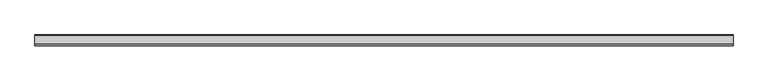
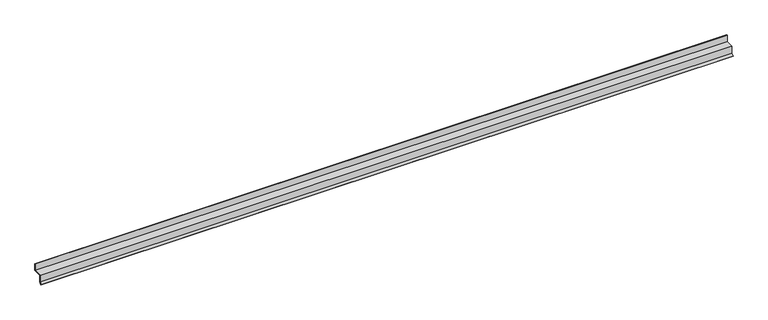
"""IFC4 building model written with IfcOpenShell, lengths in millimetres: proxy geometry, Generic Models 7:Generic Models 1:337419:Generic Models 1:337419 : Generic Models 7:Generic Models 1:337419:7 : Generic Models 7:Generic Models 1:337419:Generic Models 1:337419 : Generic Models 7:Generic Models 1:337419:301336."""

import ifcopenshell
import ifcopenshell.guid

model = None  # the IFC model being written
_history = None  # IfcOwnerHistory: only IFC2X3 demands one
_inside = {}  # id of a spatial element -> (the spatial element, [elements in it])
_under = {}  # id of a project, library or spatial element -> (it, [spatial elements below it])
_declared = {}  # id of a project -> (the project, [libraries it declares])
_typed = {}  # id of a type object -> (the type object, [elements of that type])
_made_of = {}  # id of a material, layer set ... -> (it, [elements and type objects made of it])


def new_model(schema):
    """Start an empty IFC model of exactly this schema.

    Asked for "IFC4X3", IfcOpenShell would pick the latest addendum, in which some entities
    have other attributes; the version numbers below select the first issue.
    IFC2X3 requires an IfcOwnerHistory on every rooted entity: one is made here for all.
    """
    global model, _history
    if schema == "IFC4X3":
        model = ifcopenshell.file(schema_version=(4, 3, 0, 0))
    else:
        model = ifcopenshell.file(schema=schema)
    _inside.clear()
    _under.clear()
    _declared.clear()
    _typed.clear()
    _made_of.clear()
    _history = None
    if model.schema == "IFC2X3":
        org = make("IfcOrganization", Name="unknown")
        user = make(
            "IfcPersonAndOrganization",
            ThePerson=make("IfcPerson", FamilyName="unknown"),
            TheOrganization=org,
        )
        app = make(
            "IfcApplication",
            ApplicationDeveloper=org,
            Version="unknown",
            ApplicationFullName="unknown",
            ApplicationIdentifier="unknown",
        )
        _history = make(
            "IfcOwnerHistory",
            OwningUser=user,
            OwningApplication=app,
            ChangeAction="ADDED",
            CreationDate=0,
        )
    return model


def make(cls, **values):
    """One entity of the class cls with the attributes given. An attribute that is None is left unset."""
    return model.create_entity(
        cls, **{name: value for name, value in values.items() if value is not None}
    )


def rooted(cls, **values):
    """An entity with a GlobalId (a new one), such as an element, a storey or a relation."""
    return make(cls, GlobalId=ifcopenshell.guid.new(), OwnerHistory=_history, **values)


def si_unit(unit_type, name, prefix=None):
    """IfcSIUnit, for example si_unit("LENGTHUNIT", "METRE", prefix="MILLI")."""
    return make("IfcSIUnit", UnitType=unit_type, Prefix=prefix, Name=name)


def assignment(units):
    """IfcUnitAssignment: the units of a project."""
    return None if units is None else make("IfcUnitAssignment", Units=units)


def point(xyz):
    """IfcCartesianPoint."""
    return None if xyz is None else make("IfcCartesianPoint", Coordinates=xyz)


def direction(xyz):
    """IfcDirection."""
    return None if xyz is None else make("IfcDirection", DirectionRatios=xyz)


def frame(location, z_axis=None, x_axis=None):
    """IfcAxis2Placement3D, a coordinate frame: its origin and axes. An axis left out is left unset."""
    return make(
        "IfcAxis2Placement3D",
        Location=point(location),
        Axis=direction(z_axis),
        RefDirection=direction(x_axis),
    )


def origin():
    """The frame at (0, 0, 0) with its axes left unset."""
    return frame((0.0, 0.0, 0.0))


def place(relative_to, where):
    """IfcLocalPlacement: puts the frame where relative to a parent placement (None: the world)."""
    return make(
        "IfcLocalPlacement", PlacementRelTo=relative_to, RelativePlacement=where
    )


def context(
    kind, dimensions, precision=None, world=None, true_north=None, identifier=None
):
    """IfcGeometricRepresentationContext, for example the 3D "Model" context."""
    return make(
        "IfcGeometricRepresentationContext",
        ContextIdentifier=identifier,
        ContextType=kind,
        CoordinateSpaceDimension=dimensions,
        Precision=precision,
        WorldCoordinateSystem=world,
        TrueNorth=true_north,
    )


def project(units=None, contexts=None):
    """IfcProject with its units and contexts."""
    return rooted(
        "IfcProject",
        Name="project",
        RepresentationContexts=contexts,
        UnitsInContext=assignment(units),
    )


def spatial(cls, under=None, at=None, **own):
    """A site, building, storey or space (cls), placed at a placement, below another one or the project."""
    s = rooted(cls, ObjectPlacement=at, **own)
    if under is not None:
        _under.setdefault(under.id(), (under, []))[1].append(s)
    return s


def polyline(points):
    """IfcPolyline through the points."""
    return make("IfcPolyline", Points=[point(p) for p in points])


def outline(outer, holes=None, kind="AREA"):
    """IfcArbitraryClosedProfileDef: a profile drawn as a closed curve; with holes, ...WithVoids."""
    if holes is None:
        return make("IfcArbitraryClosedProfileDef", ProfileType=kind, OuterCurve=outer)
    return make(
        "IfcArbitraryProfileDefWithVoids",
        ProfileType=kind,
        OuterCurve=outer,
        InnerCurves=holes,
    )


def extrude(swept, where, along, depth):
    """IfcExtrudedAreaSolid: the profile swept, set in the frame where, extruded along a direction by depth."""
    return make(
        "IfcExtrudedAreaSolid",
        SweptArea=swept,
        Position=where,
        ExtrudedDirection=direction(along),
        Depth=depth,
    )


def shape(context_of_items, identifier, shape_type, items):
    """IfcShapeRepresentation: the items that make up one representation, for example the "Body"."""
    return make(
        "IfcShapeRepresentation",
        ContextOfItems=context_of_items,
        RepresentationIdentifier=identifier,
        RepresentationType=shape_type,
        Items=items,
    )


def source(mapping_origin, context_of_items, identifier, shape_type, items):
    """IfcRepresentationMap: a shape defined once, which mapped items show again and again."""
    return make(
        "IfcRepresentationMap",
        MappingOrigin=mapping_origin,
        MappedRepresentation=shape(context_of_items, identifier, shape_type, items),
    )


def transform(
    local_origin,
    x_axis=None,
    y_axis=None,
    z_axis=None,
    scale=None,
    scale2=None,
    scale3=None,
    uniform=True,
):
    """IfcCartesianTransformationOperator3D, or its non-uniform kind. x_axis, y_axis, z_axis: its Axis1, 2, 3."""
    if uniform:
        return make(
            "IfcCartesianTransformationOperator3D",
            Axis1=direction(x_axis),
            Axis2=direction(y_axis),
            LocalOrigin=point(local_origin),
            Scale=scale,
            Axis3=direction(z_axis),
        )
    return make(
        "IfcCartesianTransformationOperator3DnonUniform",
        Axis1=direction(x_axis),
        Axis2=direction(y_axis),
        LocalOrigin=point(local_origin),
        Scale=scale,
        Axis3=direction(z_axis),
        Scale2=scale2,
        Scale3=scale3,
    )


def mapped(mapping_source, mapping_target):
    """IfcMappedItem: shows the shape of a source again, moved by a transform."""
    return make(
        "IfcMappedItem", MappingSource=mapping_source, MappingTarget=mapping_target
    )


def made_of(thing, what):
    """Note that an element or type object is made of a material, layer set ...; save() writes the relation."""
    if what is not None:
        _made_of.setdefault(what.id(), (what, []))[1].append(thing)
    return thing


def element(
    cls,
    number,
    at=None,
    inside=None,
    cuts=None,
    type_object=None,
    material=None,
    context=None,
    identifier="Body",
    shape_type=None,
    held_by="IfcProductDefinitionShape",
    body=None,
    shapes=None,
    **own,
):
    """One element of the class cls, such as IfcWall. Its Tag is "e" and its number.

    at: its placement. inside: the storey or other place that contains it. cuts: it is an
    opening in that element (IfcRelVoidsElement). A single representation is given by context,
    identifier, shape_type and body (its items); several are given by shapes. held_by: the class
    of the entity that holds the representations. save() writes the other relations.
    """
    e = rooted(cls, Tag="e%d" % number, ObjectPlacement=at, **own)
    if body is not None:
        shapes = [shape(context, identifier, shape_type, body)]
    if shapes is not None:
        e.Representation = make(held_by, Representations=shapes)
    if inside is not None:
        _inside.setdefault(inside.id(), (inside, []))[1].append(e)
    if cuts is not None:
        rooted(
            "IfcRelVoidsElement", RelatingBuildingElement=cuts, RelatedOpeningElement=e
        )
    if type_object is not None:
        _typed.setdefault(type_object.id(), (type_object, []))[1].append(e)
    return made_of(e, material)


def aggregate(whole, parts):
    """IfcRelAggregates: a whole, such as a stair, and the parts it consists of."""
    return rooted("IfcRelAggregates", RelatingObject=whole, RelatedObjects=parts)


def save(model, path):
    """Write the relations noted so far, then the file.

    IfcRelAggregates (storeys below a building ...), IfcRelContainedInSpatialStructure (elements
    in a storey), IfcRelDefinesByType, IfcRelAssociatesMaterial and IfcRelDeclares: one each for
    every whole, place, type object, material and project.
    """
    for whole, parts in _under.values():
        aggregate(whole, parts)
    for where, things in _inside.values():
        rooted(
            "IfcRelContainedInSpatialStructure",
            RelatedElements=things,
            RelatingStructure=where,
        )
    for kind, things in _typed.values():
        rooted("IfcRelDefinesByType", RelatedObjects=things, RelatingType=kind)
    for what, things in _made_of.values():
        rooted("IfcRelAssociatesMaterial", RelatedObjects=things, RelatingMaterial=what)
    for by, libraries in _declared.values():
        rooted("IfcRelDeclares", RelatingContext=by, RelatedDefinitions=libraries)
    model.write(path)


def generic_models_4a6affe0(model_context):
    return source(origin(), model_context, "Body", "SweptSolid", [
        extrude(outline(polyline([(-568211.286182, 4851.0990819), (-568271.214307, 4851.0990819), (-568271.214307, 4801.9264699), (-568285.4983852, 4787.6423917), (-568287.4628162, 4789.6068227), (-568273.992432, 4803.0772069), (-568273.992432, 4853.8772069), (-568214.064307, 4853.8772069), (-568214.064307, 4901.8990819), (-568211.286182, 4901.8990819), (-568211.286182, 4851.0990819)])), frame((591306.0367242, 0.0, 0.0), z_axis=(1.0, 0.0, 0.0), x_axis=(0.0, 1.0, 0.0)), (0.0, 0.0, 1.0), 4876.8),
    ])


if __name__ == "__main__":
    model = new_model("IFC4")
    model_context = context("Model", 3, world=origin())
    ifc_project = project(units=[si_unit("LENGTHUNIT", "METRE", prefix="MILLI")], contexts=[model_context])
    site = spatial("IfcSite", under=ifc_project)
    building = spatial("IfcBuilding", under=site)
    placement = place(None, origin())
    generic_models_shape = generic_models_4a6affe0(model_context)
    element("IfcBuildingElementProxy", 1, Name="Generic Models 7:Generic Models 1:337419:Generic Models 1:337419 : Generic Models 7:Generic Models 1:337419:7 : Generic Models 7:Generic Models 1:337419:Generic Models 1:337419 : Generic Models 7:Generic Models 1:337419:301336", ObjectType="Generic Models 7:Generic Models 1:337419:Generic Models 1:337419 : Generic Models 7:Generic Models 1:337419:7 : Generic Models 7:Generic Models 1:337419:Generic Models 1:337419 : Generic Models 7:Generic Models 1:337419:301336", at=placement, inside=building, context=model_context, shape_type="MappedRepresentation", body=[
        mapped(generic_models_shape, transform((0.0, 0.0, 0.0), x_axis=(1.0, 0.0, 0.0), y_axis=(0.0, 1.0, 0.0), z_axis=(0.0, 0.0, 1.0))),
    ])
    save(model, "model.ifc")

# Revit data of these elements
# Type "Generic Models 7:Generic Models 1:337419:Generic Models 1:337419 : Generic Models 7:Generic Models 1:337419:7 : Generic Models 7:Generic Models 1:337419:Generic Models 1:337419 : Generic Models 7:Generic Models 1:337419:301336"
#   NameOverride = "Generic Models 7:Generic Models 1:337419:Generic Models 1:337419 : Generic Models 7:Generic Models 1:337419:301336"
#   ObjectTypeOverride = "Generic Models 1:337419 : Generic Models 7:Generic Models 1:337419"
#   Reference = "Generic Models 1"
#   Tag = "301336"
# Element 1 (IfcBuildingElementProxy, "Generic Models 7:Generic Models 1:337419:Generic Models 1:337419 : Generic Models 7:Generic Models 1:337419:7 : Generic Models 7:Generic Models 1:337419:Generic Models 1:337419 : Generic Models 7:Generic Models 1:337419:301336")
#   Materials on its faces: "BRAKE METAL FLASHING"
# Materials
#   "BRAKE METAL FLASHING": class "Unassigned", colour RGB 210 209 208, transparency 0, Cost = 0
